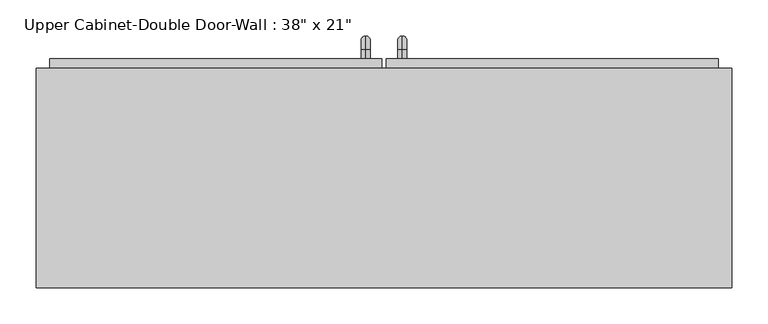
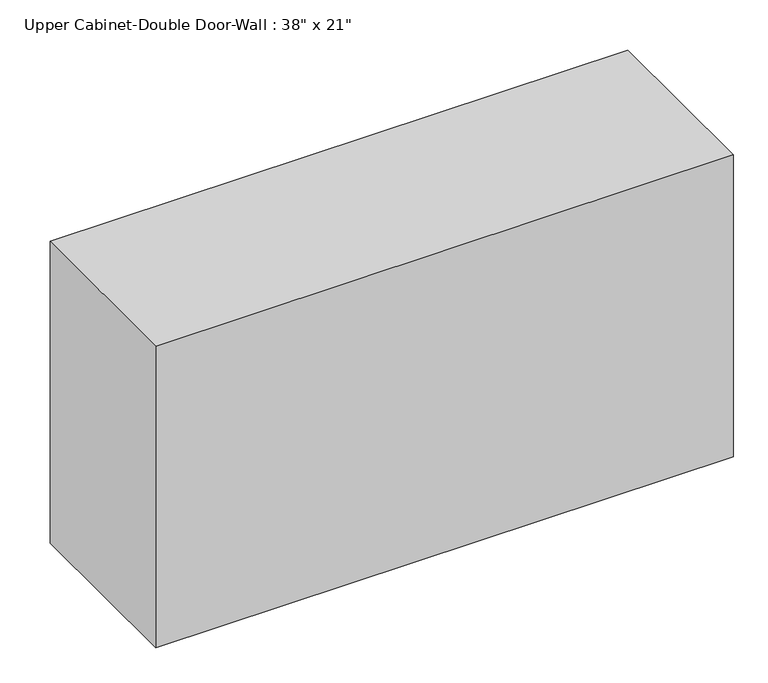
"""IFC4 building model written with IfcOpenShell, lengths in millimetres: furniture geometry."""

from ifc_helpers import new_model, si_unit, point, frame, origin, place, context, project, spatial, polyline, circle_curve, ellipse_curve, trimmed, outline, extrude, faceted_brep, source, transform, mapped, element, save
from ifc_brep_helpers import plane_surface, cylinder_surface, revolved_surface, advanced_brep


def furniture_06efdd11(model_context):
    return source(origin(), model_context, "Body", "SolidModel", [
        faceted_brep([(-452.8288372, 61.9125, 2438.4), (-452.8288372, 61.9125, 1905.0), (512.3711628, 61.9125, 1905.0), (512.3711628, 61.9125, 2438.4), (-452.8288372, 366.7125, 2438.4), (512.3711628, 366.7125, 2438.4), (512.3711628, 366.7125, 1905.0), (-452.8288372, 366.7125, 1905.0), (-433.7788372, 366.7125, 2419.35), (-433.7788372, 366.7125, 1924.05), (493.3211628, 366.7125, 1924.05), (493.3211628, 366.7125, 2419.35), (493.3211628, 80.9625, 2419.35), (-433.7788372, 80.9625, 2419.35), (493.3211628, 80.9625, 1924.05), (-433.7788372, 80.9625, 1924.05)], [[[0, 1, 2, 3]], [[4, 5, 6, 7], [8, 9, 10, 11]], [[1, 0, 4, 7]], [[2, 1, 7, 6]], [[3, 2, 6, 5]], [[0, 3, 5, 4]], [[8, 11, 12, 13]], [[11, 10, 14, 12]], [[10, 9, 15, 14]], [[9, 8, 13, 15]], [[13, 12, 14, 15]]]),
        advanced_brep(
        [(55.1711628, 379.4125, 2051.05), (55.1711628, 379.4125, 2063.75), (55.1711628, 392.1125, 2051.05), (55.1711628, 392.1125, 2063.75), (55.1711628, 411.1625, 2044.7), (55.1711628, 398.4625, 2044.7), (55.1711628, 398.4625, 1968.5), (55.1711628, 411.1625, 1968.5), (55.1711628, 392.1125, 1949.45), (55.1711628, 392.1125, 1962.15), (55.1711628, 379.4125, 1962.15), (55.1711628, 379.4125, 1949.45)],
        [
            (0, 1, circle_curve(frame((55.1711628, 379.4125, 2057.4), z_axis=(0.0, -1.0, 0.0), x_axis=(0.0, 0.0, -1.0)), 6.35)),
            (1, 0, circle_curve(frame((55.1711628, 379.4125, 2057.4), z_axis=(0.0, -1.0, 0.0), x_axis=(0.0, 0.0, -1.0)), 6.35)),
            (0, 2),
            (2, 3, circle_curve(frame((55.1711628, 392.1125, 2057.4), z_axis=(0.0, -1.0, 0.0), x_axis=(0.0, 0.0, -1.0)), 6.35)),
            (3, 1),
            (3, 2, circle_curve(frame((55.1711628, 392.1125, 2057.4), z_axis=(0.0, -1.0, 0.0), x_axis=(0.0, 0.0, -1.0)), 6.35)),
            (4, 3, circle_curve(frame((55.1711628, 392.1125, 2044.7), z_axis=(1.0, 0.0, 0.0), x_axis=(0.0, 0.0, 1.0)), 19.05)),
            (2, 5, circle_curve(frame((55.1711628, 392.1125, 2044.7), z_axis=(-1.0, 0.0, 0.0), x_axis=(0.0, 0.0, 1.0)), 6.35)),
            (5, 4, circle_curve(frame((55.1711628, 404.8125, 2044.7), z_axis=(0.0, 0.0, 1.0), x_axis=(0.0, -1.0, 0.0)), 6.35)),
            (4, 5, circle_curve(frame((55.1711628, 404.8125, 2044.7), z_axis=(0.0, 0.0, 1.0), x_axis=(0.0, -1.0, 0.0)), 6.35)),
            (5, 6),
            (6, 7, circle_curve(frame((55.1711628, 404.8125, 1968.5), z_axis=(0.0, 0.0, 1.0), x_axis=(0.0, -1.0, 0.0)), 6.35)),
            (7, 4),
            (7, 6, circle_curve(frame((55.1711628, 404.8125, 1968.5), z_axis=(0.0, 0.0, 1.0), x_axis=(0.0, -1.0, 0.0)), 6.35)),
            (8, 7, circle_curve(frame((55.1711628, 392.1125, 1968.5), z_axis=(1.0, 0.0, 0.0), x_axis=(0.0, 1.0, 0.0)), 19.05)),
            (6, 9, circle_curve(frame((55.1711628, 392.1125, 1968.5), z_axis=(-1.0, 0.0, 0.0), x_axis=(0.0, 1.0, 0.0)), 6.35)),
            (9, 8, circle_curve(frame((55.1711628, 392.1125, 1955.8), z_axis=(0.0, 1.0, 0.0), x_axis=(0.0, 0.0, 1.0)), 6.35)),
            (8, 9, circle_curve(frame((55.1711628, 392.1125, 1955.8), z_axis=(0.0, 1.0, 0.0), x_axis=(0.0, 0.0, 1.0)), 6.35)),
            (10, 11, circle_curve(frame((55.1711628, 379.4125, 1955.8), z_axis=(0.0, -1.0, 0.0), x_axis=(0.0, 0.0, 1.0)), 6.35)),
            (11, 10, circle_curve(frame((55.1711628, 379.4125, 1955.8), z_axis=(0.0, -1.0, 0.0), x_axis=(0.0, 0.0, 1.0)), 6.35)),
            (9, 10),
            (11, 8),
        ],
        [
            plane_surface(frame((48.8211628, 379.4125, 2057.4), z_axis=(0.0, -1.0, 0.0), x_axis=(0.0, 0.0, 1.0))),
            cylinder_surface(frame((55.1711628, 379.4125, 2057.4), z_axis=(0.0, -1.0, 0.0), x_axis=(0.0, 0.0, -1.0)), 6.35),
            revolved_surface(trimmed(ellipse_curve(frame((55.1711628, 392.1125, 2057.4), z_axis=(0.0, -1.0, 0.0), x_axis=(0.0, 0.0, -1.0)), 6.35, 6.35), [point((55.1711628, 392.1125, 2051.05))], [point((55.1711628, 392.1125, 2063.75))], True, "CARTESIAN"), (55.1711628, 392.1125, 2044.7), (-1.0, 0.0, 0.0)),
            revolved_surface(trimmed(ellipse_curve(frame((55.1711628, 392.1125, 2057.4), z_axis=(0.0, -1.0, 0.0), x_axis=(0.0, 0.0, -1.0)), 6.35, 6.35), [point((55.1711628, 392.1125, 2063.75))], [point((55.1711628, 392.1125, 2051.05))], True, "CARTESIAN"), (55.1711628, 392.1125, 2044.7), (-1.0, 0.0, 0.0)),
            cylinder_surface(frame((55.1711628, 404.8125, 2044.7), z_axis=(0.0, 0.0, 1.0), x_axis=(0.0, -1.0, 0.0)), 6.35),
            revolved_surface(trimmed(ellipse_curve(frame((55.1711628, 404.8125, 1968.5), z_axis=(0.0, 0.0, 1.0), x_axis=(0.0, -1.0, 0.0)), 6.35, 6.35), [point((55.1711628, 398.4625, 1968.5))], [point((55.1711628, 411.1625, 1968.5))], True, "CARTESIAN"), (55.1711628, 392.1125, 1968.5), (-1.0, 0.0, 0.0)),
            revolved_surface(trimmed(ellipse_curve(frame((55.1711628, 404.8125, 1968.5), z_axis=(0.0, 0.0, 1.0), x_axis=(0.0, -1.0, 0.0)), 6.35, 6.35), [point((55.1711628, 411.1625, 1968.5))], [point((55.1711628, 398.4625, 1968.5))], True, "CARTESIAN"), (55.1711628, 392.1125, 1968.5), (-1.0, 0.0, 0.0)),
            plane_surface(frame((48.8211628, 379.4125, 1955.8), z_axis=(0.0, -1.0, 0.0), x_axis=(0.0, 0.0, -1.0))),
            cylinder_surface(frame((55.1711628, 392.1125, 1955.8), z_axis=(0.0, 1.0, 0.0), x_axis=(0.0, 0.0, 1.0)), 6.35),
        ],
        [
            (0, [[1, 2]]),
            (1, [[-1, 3, 4, 5]]),
            (1, [[-2, -5, 6, -3]]),
            (2, [[7, -4, 8, 9]]),
            (3, [[-8, -6, -7, 10]]),
            (4, [[-9, 11, 12, 13]]),
            (4, [[-10, -13, 14, -11]]),
            (5, [[15, -12, 16, 17]]),
            (6, [[-16, -14, -15, 18]]),
            (7, [[19, 20]]),
            (8, [[-17, 21, -20, 22]]),
            (8, [[-18, -22, -19, -21]]),
        ],
    ),
        advanced_brep(
        [(4.3711628, 379.4125, 2051.05), (4.3711628, 379.4125, 2063.75), (4.3711628, 392.1125, 2051.05), (4.3711628, 392.1125, 2063.75), (4.3711628, 411.1625, 2044.7), (4.3711628, 398.4625, 2044.7), (4.3711628, 398.4625, 1968.5), (4.3711628, 411.1625, 1968.5), (4.3711628, 392.1125, 1949.45), (4.3711628, 392.1125, 1962.15), (4.3711628, 379.4125, 1962.15), (4.3711628, 379.4125, 1949.45)],
        [
            (0, 1, circle_curve(frame((4.3711628, 379.4125, 2057.4), z_axis=(0.0, -1.0, 0.0), x_axis=(0.0, 0.0, 1.0)), 6.35)),
            (1, 0, circle_curve(frame((4.3711628, 379.4125, 2057.4), z_axis=(0.0, -1.0, 0.0), x_axis=(0.0, 0.0, 1.0)), 6.35)),
            (0, 2),
            (2, 3, circle_curve(frame((4.3711628, 392.1125, 2057.4), z_axis=(0.0, -1.0, 0.0), x_axis=(0.0, 0.0, 1.0)), 6.35)),
            (3, 1),
            (3, 2, circle_curve(frame((4.3711628, 392.1125, 2057.4), z_axis=(0.0, -1.0, 0.0), x_axis=(0.0, 0.0, 1.0)), 6.35)),
            (4, 3, circle_curve(frame((4.3711628, 392.1125, 2044.7), z_axis=(1.0, 0.0, 0.0), x_axis=(0.0, 0.0, 1.0)), 19.05)),
            (2, 5, circle_curve(frame((4.3711628, 392.1125, 2044.7), z_axis=(-1.0, 0.0, 0.0), x_axis=(0.0, 0.0, 1.0)), 6.35)),
            (5, 4, circle_curve(frame((4.3711628, 404.8125, 2044.7), z_axis=(0.0, 0.0, 1.0), x_axis=(0.0, 1.0, 0.0)), 6.35)),
            (4, 5, circle_curve(frame((4.3711628, 404.8125, 2044.7), z_axis=(0.0, 0.0, 1.0), x_axis=(0.0, 1.0, 0.0)), 6.35)),
            (5, 6),
            (6, 7, circle_curve(frame((4.3711628, 404.8125, 1968.5), z_axis=(0.0, 0.0, 1.0), x_axis=(0.0, 1.0, 0.0)), 6.35)),
            (7, 4),
            (7, 6, circle_curve(frame((4.3711628, 404.8125, 1968.5), z_axis=(0.0, 0.0, 1.0), x_axis=(0.0, 1.0, 0.0)), 6.35)),
            (8, 7, circle_curve(frame((4.3711628, 392.1125, 1968.5), z_axis=(1.0, 0.0, 0.0), x_axis=(0.0, 1.0, 0.0)), 19.05)),
            (6, 9, circle_curve(frame((4.3711628, 392.1125, 1968.5), z_axis=(-1.0, 0.0, 0.0), x_axis=(0.0, 1.0, 0.0)), 6.35)),
            (9, 8, circle_curve(frame((4.3711628, 392.1125, 1955.8), z_axis=(0.0, 1.0, 0.0), x_axis=(0.0, 0.0, -1.0)), 6.35)),
            (8, 9, circle_curve(frame((4.3711628, 392.1125, 1955.8), z_axis=(0.0, 1.0, 0.0), x_axis=(0.0, 0.0, -1.0)), 6.35)),
            (10, 11, circle_curve(frame((4.3711628, 379.4125, 1955.8), z_axis=(0.0, -1.0, 0.0), x_axis=(0.0, 0.0, -1.0)), 6.35)),
            (11, 10, circle_curve(frame((4.3711628, 379.4125, 1955.8), z_axis=(0.0, -1.0, 0.0), x_axis=(0.0, 0.0, -1.0)), 6.35)),
            (9, 10),
            (11, 8),
        ],
        [
            plane_surface(frame((-1.9788372, 379.4125, 2057.4), z_axis=(0.0, -1.0, 0.0), x_axis=(0.0, 0.0, 1.0))),
            cylinder_surface(frame((4.3711628, 379.4125, 2057.4), z_axis=(0.0, -1.0, 0.0), x_axis=(0.0, 0.0, 1.0)), 6.35),
            revolved_surface(trimmed(ellipse_curve(frame((4.3711628, 392.1125, 2057.4), z_axis=(0.0, -1.0, 0.0), x_axis=(0.0, 0.0, 1.0)), 6.35, 6.35), [point((4.3711628, 392.1125, 2051.05))], [point((4.3711628, 392.1125, 2063.75))], True, "CARTESIAN"), (4.3711628, 392.1125, 2044.7), (-1.0, 0.0, 0.0)),
            revolved_surface(trimmed(ellipse_curve(frame((4.3711628, 392.1125, 2057.4), z_axis=(0.0, -1.0, 0.0), x_axis=(0.0, 0.0, 1.0)), 6.35, 6.35), [point((4.3711628, 392.1125, 2063.75))], [point((4.3711628, 392.1125, 2051.05))], True, "CARTESIAN"), (4.3711628, 392.1125, 2044.7), (-1.0, 0.0, 0.0)),
            cylinder_surface(frame((4.3711628, 404.8125, 2044.7), z_axis=(0.0, 0.0, 1.0), x_axis=(0.0, 1.0, 0.0)), 6.35),
            revolved_surface(trimmed(ellipse_curve(frame((4.3711628, 404.8125, 1968.5), z_axis=(0.0, 0.0, 1.0), x_axis=(0.0, 1.0, 0.0)), 6.35, 6.35), [point((4.3711628, 398.4625, 1968.5))], [point((4.3711628, 411.1625, 1968.5))], True, "CARTESIAN"), (4.3711628, 392.1125, 1968.5), (-1.0, 0.0, 0.0)),
            revolved_surface(trimmed(ellipse_curve(frame((4.3711628, 404.8125, 1968.5), z_axis=(0.0, 0.0, 1.0), x_axis=(0.0, 1.0, 0.0)), 6.35, 6.35), [point((4.3711628, 411.1625, 1968.5))], [point((4.3711628, 398.4625, 1968.5))], True, "CARTESIAN"), (4.3711628, 392.1125, 1968.5), (-1.0, 0.0, 0.0)),
            plane_surface(frame((-1.9788372, 379.4125, 1955.8), z_axis=(0.0, -1.0, 0.0), x_axis=(0.0, 0.0, -1.0))),
            cylinder_surface(frame((4.3711628, 392.1125, 1955.8), z_axis=(0.0, 1.0, 0.0), x_axis=(0.0, 0.0, -1.0)), 6.35),
        ],
        [
            (0, [[1, 2]]),
            (1, [[-1, 3, 4, 5]]),
            (1, [[-2, -5, 6, -3]]),
            (2, [[7, -4, 8, 9]]),
            (3, [[-8, -6, -7, 10]]),
            (4, [[-9, 11, 12, 13]]),
            (4, [[-10, -13, 14, -11]]),
            (5, [[15, -12, 16, 17]]),
            (6, [[-16, -14, -15, 18]]),
            (7, [[19, 20]]),
            (8, [[-17, 21, -20, 22]]),
            (8, [[-18, -22, -19, -21]]),
        ],
    ),
        extrude(outline(polyline([(32.9461628, 379.4125), (493.3211628, 379.4125), (493.3211628, 347.6625), (32.9461628, 347.6625), (32.9461628, 379.4125)])), frame((0.0, 0.0, 1924.05), z_axis=(0.0, 0.0, 1.0), x_axis=(1.0, 0.0, 0.0)), (0.0, 0.0, 1.0), 495.3),
        extrude(outline(polyline([(-433.7788372, 379.4125), (26.5961628, 379.4125), (26.5961628, 347.6625), (-433.7788372, 347.6625), (-433.7788372, 379.4125)])), frame((0.0, 0.0, 1924.05), z_axis=(0.0, 0.0, 1.0), x_axis=(1.0, 0.0, 0.0)), (0.0, 0.0, 1.0), 495.3),
    ])


if __name__ == "__main__":
    model = new_model("IFC4")
    model_context = context("Model", 3, world=origin())
    ifc_project = project(units=[si_unit("LENGTHUNIT", "METRE", prefix="MILLI")], contexts=[model_context])
    site = spatial("IfcSite", under=ifc_project)
    building = spatial("IfcBuilding", under=site)
    placement = place(None, origin())
    furniture_shape = furniture_06efdd11(model_context)
    element("IfcFurniture", 1, ObjectType="Upper Cabinet-Double Door-Wall : 38\" x 21\"", at=placement, inside=building, context=model_context, shape_type="MappedRepresentation", body=[
        mapped(furniture_shape, transform((0.0, 0.0, 0.0), x_axis=(1.0, 0.0, 0.0), y_axis=(0.0, 1.0, 0.0), z_axis=(0.0, 0.0, 1.0))),
    ])
    save(model, "model.ifc")

# Revit data of these elements
# Type "Upper Cabinet-Double Door-Wall : 38\" x 21\""
#   COBie.Type.CreatedBy = "doug.wood@us.ibm.com"
#   COBie.Type.CreatedOn = "2016-04-14T02:07:23"
#   COBie.Type.Name = "Casework_Upper Cabinet-Double Door-Wall_38\" x 21\""
#   COBie.Type.Category = "23-40 35 17 47 11 : Kitchen Casework"
#   COBie.Type.Description = "Upper Cabinet-Double Door-Wall_38\" x 21\""
#   COBie.Type.Manufacturer = ""
#   COBie.Type.ModelNumber = ""
#   Assembly Code = "C1030410"
#   COBie.Type.ReplacementCost = 0
#   Depth = 1' - 0"
#   Height = 1' - 9"
#   Top Of Cabinet = 8' - 0"
#   Width = 3' - 2"
#   COBie.Type = no
#   Cabinet Material = none
#   Door/Drawer Material = none
#   Handle Material = Cabinets - Handles
# Element 1 (IfcFurniture, "Upper Cabinet-Double Door-Wall : 38\" x 21\"")
#   Materials on its faces: "Cabinets - Handles", "Cabinets"
# Materials
#   "Cabinets - Handles": class "Metal", colour RGB 57 57 57, transparency 0
#   "Cabinets": class "Miscellaneous", colour RGB 249 249 249, transparency 0
